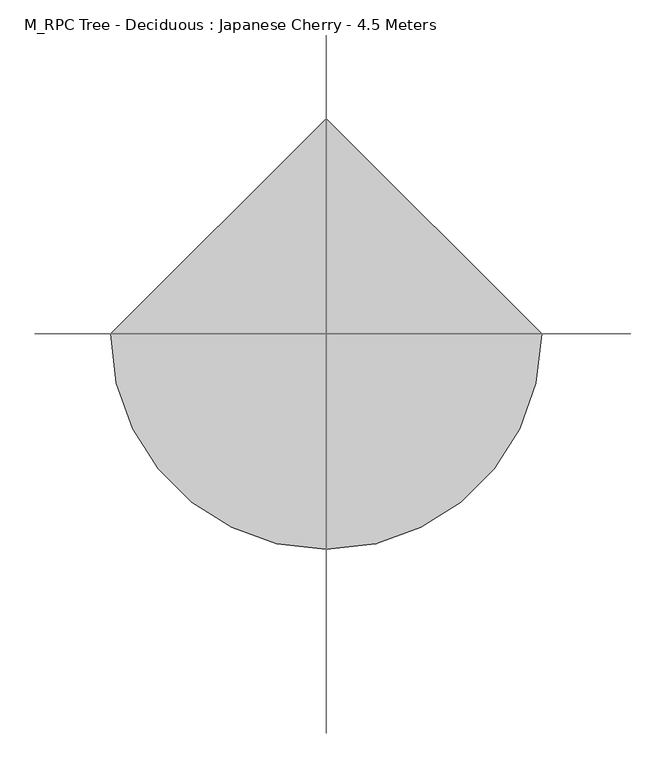
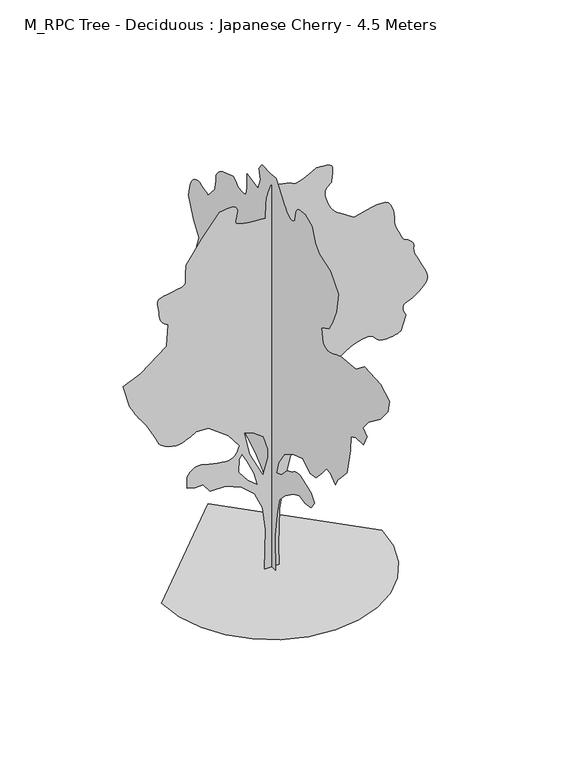
"""IFC4 building model written with IfcOpenShell, lengths in millimetres: geographic element geometry, M_RPC Tree - Deciduous : Japanese Cherry - 4.5 Meters."""

from ifc_helpers import new_model, si_unit, origin, place, context, project, spatial, triangles, source, transform, mapped, element, save


def m_rpc_tree_deciduous_japanese_cherry_4_5_meters_cd2ce576(model_context):
    return source(origin(), model_context, "Body", "Tessellation", [
        triangles([(-0.0027587, 74.5725603, 0.00586), (-0.0027587, -72.0943095, 0.00586), (-0.0027587, -58.7610481, 393.3378007), (-0.0027587, -98.7608322, 653.338028), (-0.0027587, -145.4276149, 853.3381748), (-0.0027587, -252.0952047, 966.670792), (-0.0027587, -412.0928332, 1080.00588), (-0.0027587, -518.7604139, 1126.6709095), (-0.0027587, -625.428031, 1106.6708948), (-0.0027587, -738.7605755, 1126.6709095), (-0.0027587, -798.7606195, 1213.3384392), (-0.0027587, -738.7605755, 1293.3384979), (-0.0027587, -525.4279212, 1366.6710857), (-0.0027587, -506.885412, 1365.1761189), (-0.0027587, -488.5178922, 1363.2711479), (-0.0027587, -470.5003873, 1360.5486397), (-0.0027587, -453.0078504, 1356.6035316), (-0.0027587, -436.2153434, 1351.0261105), (-0.0027587, -420.2953485, 1343.4060814), (-0.0027587, -405.4278331, 1333.3385273), (-0.0027587, -390.5578105, 1322.4935497), (-0.0027587, -374.6402864, 1312.6960373), (-0.0027587, -357.8477795, 1303.7760876), (-0.0027587, -340.3552789, 1295.553479), (-0.0027587, -322.337774, 1287.8585999), (-0.0027587, -303.970236, 1280.5110832), (-0.0027587, -285.4277268, 1273.3385559), (-0.0027587, -185.427399, 1166.6709389), (-0.0027587, -85.4275708, 1126.6709095), (-0.0027587, -125.4276002, 1266.671085), (-0.0027587, -238.7606988, 1433.3386734), (-0.0027587, -398.7603258, 1533.3386742), (-0.0027587, -585.4279653, 1593.3387909), (-0.0027587, -718.7605608, 1506.6712612), (-0.0027587, -825.4281778, 1520.0062031), (-0.0027587, -938.7607224, 1640.0038204), (-0.0027587, -1025.4283247, 1746.6714375), (-0.0027587, -1105.4259127, 1740.0038212), (-0.0027587, -1192.0934423, 1660.0063786), (-0.0027587, -1245.4260155, 1753.3389084), (-0.0027587, -1305.4259869, 1820.0040253), (-0.0027587, -1412.0936039, 1933.3391132), (-0.0027587, -1478.7587208, 2233.3392609), (-0.0027587, -1485.4261917, 2393.3393784), (-0.0027587, -1578.7611923, 2433.336937), (-0.0027587, -1725.426368, 2446.6718788), (-0.0027587, -1785.4264847, 2573.3269386), (-0.0027587, -1712.0938969, 2633.3270554), (-0.0027587, -1812.0938976, 2753.3272888), (-0.0027587, -2038.759132, 2926.6774635), (-0.0027587, -2185.4267784, 3100.0023491), (-0.0027587, -2212.0917206, 3240.0025246), (-0.0027587, -2045.4266029, 3333.3276421), (-0.0027587, -1738.758839, 3346.6776993), (-0.0027587, -1585.4263378, 3226.6774658), (-0.0027587, -1292.0935158, 3193.3274666), (-0.0027587, -1252.2485641, 3177.7025482), (-0.0027587, -1213.3384392, 3162.6025978), (-0.0027587, -1176.2909185, 3148.5525833), (-0.0027587, -1142.0459158, 3136.0774727), (-0.0027587, -1111.5309179, 3125.7025246), (-0.0027587, -1085.6808969, 3117.9524162), (-0.0027587, -1065.4258833, 3113.3274078), (-0.0027587, -1047.2933418, 3113.0774231), (-0.0027587, -1028.108321, 3117.0274727), (-0.0027587, -1009.2758223, 3123.652359), (-0.0027587, -992.1908186, 3131.4524643), (-0.0027587, -978.255768, 3138.9025909), (-0.0027587, -968.8682596, 3144.4775414), (-0.0027587, -965.4257372, 3146.6774071), (-0.0027587, -932.0932514, 3306.6775246), (-0.0027587, -1072.0933542, 3380.0027), (-0.0027587, -1138.7609419, 3486.6778748), (-0.0027587, -1212.093457, 3660.003051), (-0.0027587, -1252.0934864, 3880.0029945), (-0.0027587, -1098.7609125, 4053.3281708), (-0.0027587, -898.760693, 4126.6783447), (-0.0027587, -818.7606342, 4200.0032295), (-0.0027587, -758.7605902, 4360.003347), (-0.0027587, -618.7604874, 4413.3285805), (-0.0027587, -595.9604619, 4413.2285866), (-0.0027587, -573.5129585, 4412.5536278), (-0.0027587, -551.7629416, 4410.70345), (-0.0027587, -531.0629333, 4407.1286682), (-0.0027587, -511.7629123, 4401.17845), (-0.0027587, -494.2128934, 4392.3534073), (-0.0027587, -478.7603846, 4380.0035797), (-0.0027587, -466.2228868, 4364.55336), (-0.0027587, -456.8353784, 4347.0035591), (-0.0027587, -450.0728551, 4327.7035744), (-0.0027587, -445.4078419, 4307.0033844), (-0.0027587, -442.3178415, 4285.2535492), (-0.0027587, -440.2753427, 4262.803466), (-0.0027587, -438.7603552, 4240.0034042), (-0.0027587, -427.2553525, 4227.3033073), (-0.0027587, -415.2803204, 4215.6034401), (-0.0027587, -402.3753304, 4205.9034508), (-0.0027587, -388.070317, 4199.1532814), (-0.0027587, -371.9003011, 4196.3784508), (-0.0027587, -353.3952896, 4198.553318), (-0.0027587, -332.0927745, 4206.6784035), (-0.0027587, -310.9852329, 4218.4782646), (-0.0027587, -293.0277353, 4231.0033722), (-0.0027587, -277.6927156, 4244.1034447), (-0.0027587, -264.4552061, 4257.6784882), (-0.0027587, -252.7927094, 4271.5785118), (-0.0027587, -242.1814384, 4285.7285202), (-0.0027587, -232.0939364, 4300.003521), (-0.0027587, -138.7608616, 4426.6786377), (-0.0027587, -78.7608175, 4500.0035225), (-0.0027587, 21.2393172, 4493.3286392), (-0.0027587, 181.2391372, 4500.0035225), (-0.0027587, 241.2389451, 4420.0034637), (-0.0027587, 214.5724224, 4306.6784042), (-0.0027587, 261.2402133, 4180.0032875), (-0.0027587, 467.9053785, 4220.0034622), (-0.0027587, 467.9053785, 4073.3284035), (-0.0027587, 469.4403866, 4050.6283356), (-0.0027587, 471.6178699, 4028.7032204), (-0.0027587, 475.0778695, 4008.4282951), (-0.0027587, 480.4628969, 3990.6282188), (-0.0027587, 488.4103769, 3976.0532364), (-0.0027587, 499.5679081, 3965.5782944), (-0.0027587, 514.5729152, 3960.0030533), (-0.0027587, 531.7154371, 3957.9281799), (-0.0027587, 548.8579227, 3957.2532211), (-0.0027587, 566.0004447, 3957.7281921), (-0.0027587, 583.1429667, 3959.1531052), (-0.0027587, 600.2854886, 3961.2782661), (-0.0027587, 617.4304813, 3963.853109), (-0.0027587, 634.5730396, 3966.6782272), (-0.0027587, 650.2955538, 3982.2281502), (-0.0027587, 666.0780207, 3996.928125), (-0.0027587, 681.9780676, 4009.8782066), (-0.0027587, 698.0505604, 4020.2031578), (-0.0027587, 714.3580679, 4027.0283226), (-0.0027587, 730.9580721, 4029.4781731), (-0.0027587, 747.9055841, 4026.678344), (-0.0027587, 927.9057163, 3966.6782272), (-0.0027587, 953.4457272, 3949.4781143), (-0.0027587, 977.9358021, 3931.9280228), (-0.0027587, 1000.3257872, 3913.6782646), (-0.0027587, 1019.5682899, 3894.3779892), (-0.0027587, 1034.6108311, 3873.6780899), (-0.0027587, 1044.4058001, 3851.2280067), (-0.0027587, 1047.9058044, 3826.6780518), (-0.0027587, 1048.6833733, 3801.5281334), (-0.0027587, 1050.8608566, 3777.4531494), (-0.0027587, 1054.2033125, 3754.253112), (-0.0027587, 1058.4783422, 3731.7530319), (-0.0027587, 1063.4533293, 3709.7529213), (-0.0027587, 1068.895875, 3688.1280785), (-0.0027587, 1074.570892, 3666.6779343), (-0.0027587, 1201.238451, 3526.6777588), (-0.0027587, 1239.7609543, 3543.5528915), (-0.0027587, 1277.9935043, 3558.9278252), (-0.0027587, 1315.641061, 3571.2779434), (-0.0027587, 1352.4135258, 3579.077758), (-0.0027587, 1388.0210907, 3580.8029434), (-0.0027587, 1422.1711864, 3574.9527191), (-0.0027587, 1454.5710983, 3560.0027596), (-0.0027587, 1482.6961258, 3536.9027161), (-0.0027587, 1504.8736965, 3508.1777252), (-0.0027587, 1522.093721, 3474.8027275), (-0.0027587, 1535.3487259, 3437.7026665), (-0.0027587, 1545.6312378, 3397.8027763), (-0.0027587, 1553.9313126, 3356.02771), (-0.0027587, 1561.2387154, 3313.3277), (-0.0027587, 1474.5711857, 3086.677581), (-0.0027587, 1367.9060394, 2940.0022316), (-0.0027587, 1454.5710983, 2700.0020554), (-0.0027587, 1374.5710396, 2573.3269386), (-0.0027587, 1341.9185268, 2561.8270592), (-0.0027587, 1310.4910847, 2549.851918), (-0.0027587, 1281.5110222, 2536.952124), (-0.0027587, 1256.2035553, 2522.6521248), (-0.0027587, 1235.7959347, 2506.4769493), (-0.0027587, 1221.5109055, 2487.9745903), (-0.0027587, 1214.5709948, 2466.6721115), (-0.0027587, 1212.2984591, 2444.0095413), (-0.0027587, 1211.0734612, 2421.694479), (-0.0027587, 1210.7234825, 2399.6744568), (-0.0027587, 1211.0734612, 2377.8868332), (-0.0027587, 1211.9484804, 2356.2718735), (-0.0027587, 1213.1734783, 2334.7768192), (-0.0027587, 1214.5709948, 2313.3368488), (-0.0027587, 1187.9059799, 2206.6717026), (-0.0027587, 1001.2383041, 2226.6717899), (-0.0027587, 985.728277, 2195.3792233), (-0.0027587, 971.4432478, 2164.9017231), (-0.0027587, 959.6057436, 2136.0591522), (-0.0027587, 951.4432331, 2109.6642517), (-0.0027587, 948.1782434, 2086.536739), (-0.0027587, 951.0357725, 2067.4865936), (-0.0027587, 961.2382748, 2053.3392014), (-0.0027587, 977.7782536, 2041.5990749), (-0.0027587, 998.0507807, 2029.6266953), (-0.0027587, 1020.8883402, 2018.0041489), (-0.0027587, 1045.1258142, 2007.3141037), (-0.0027587, 1069.5958323, 1998.1390823), (-0.0027587, 1093.133349, 1991.0640781), (-0.0027587, 1114.5709213, 1986.6716137), (-0.0027587, 1133.9884134, 1982.8416149), (-0.0027587, 1152.3558969, 1977.2640484), (-0.0027587, 1169.8484339, 1970.2290127), (-0.0027587, 1186.6409409, 1962.0266064), (-0.0027587, 1202.9109507, 1952.9491081), (-0.0027587, 1218.828511, 1943.2890873), (-0.0027587, 1234.5710094, 1933.3391132), (-0.0027587, 1387.9061268, 2013.339172), (-0.0027587, 1431.9861397, 2024.5916828), (-0.0027587, 1474.8436981, 2034.7965832), (-0.0027587, 1515.2512608, 2042.9016117), (-0.0027587, 1551.9862278, 2047.8566872), (-0.0027587, 1583.8238194, 2048.6141991), (-0.0027587, 1609.5388195, 2044.1266823), (-0.0027587, 1627.9038322, 2033.339114), (-0.0027587, 1640.0538174, 2017.6916679), (-0.0027587, 1648.351276, 1999.5965515), (-0.0027587, 1653.4438431, 1979.4615887), (-0.0027587, 1655.9713051, 1957.6915512), (-0.0027587, 1656.5738846, 1934.6990593), (-0.0027587, 1655.8938389, 1910.8890301), (-0.0027587, 1654.5713905, 1886.6714676), (-0.0027587, 1631.6563648, 1862.5889259), (-0.0027587, 1608.3912151, 1839.7339256), (-0.0027587, 1584.4262535, 1819.3239796), (-0.0027587, 1559.4112106, 1802.5889545), (-0.0027587, 1532.9962532, 1790.7539211), (-0.0027587, 1504.833728, 1785.038863), (-0.0027587, 1474.5711857, 1786.6714668), (-0.0027587, 1442.5211071, 1793.7065025), (-0.0027587, 1410.0036152, 1802.1439236), (-0.0027587, 1378.1860806, 1810.1114605), (-0.0027587, 1348.2360191, 1815.7489071), (-0.0027587, 1321.3160053, 1817.1864647), (-0.0027587, 1298.5960258, 1812.5614563), (-0.0027587, 1281.2385098, 1800.0039379), (-0.0027587, 1268.1185257, 1783.8339947), (-0.0027587, 1257.0985588, 1769.4114738), (-0.0027587, 1247.8260143, 1756.448893), (-0.0027587, 1239.9560005, 1744.6513573), (-0.0027587, 1233.1334518, 1733.7264427), (-0.0027587, 1227.0110058, 1723.3863762), (-0.0027587, 1221.2385384, 1713.338879), (-0.0027587, 1243.9585178, 1710.3264175), (-0.0027587, 1265.8635761, 1706.3813095), (-0.0027587, 1286.1360306, 1700.5688736), (-0.0027587, 1303.9584892, 1691.9587887), (-0.0027587, 1318.5160309, 1679.6163734), (-0.0027587, 1328.993589, 1662.608836), (-0.0027587, 1334.5710102, 1640.0038204), (-0.0027587, 1336.8460167, 1613.5137222), (-0.0027587, 1338.0710873, 1585.6212387), (-0.0027587, 1338.4210659, 1556.56371), (-0.0027587, 1338.0710873, 1526.5736801), (-0.0027587, 1337.1961407, 1495.8836929), (-0.0027587, 1335.9710701, 1464.7286179), (-0.0027587, 1334.5710102, 1433.3386734), (-0.0027587, 1300.3260075, 1407.8185741), (-0.0027587, 1266.3110779, 1383.4636654), (-0.0027587, 1232.7634163, 1361.4436432), (-0.0027587, 1199.91593, 1342.9210819), (-0.0027587, 1168.0034157, 1329.0634975), (-0.0027587, 1137.2534031, 1321.0360806), (-0.0027587, 1107.9059212, 1320.0060562), (-0.0027587, 1078.5558958, 1323.638538), (-0.0027587, 1047.808354, 1328.6735504), (-0.0027587, 1015.8932962, 1334.873608), (-0.0027587, 983.0458099, 1342.0060215), (-0.0027587, 949.4982937, 1349.8410084), (-0.0027587, 915.4857622, 1358.1386124), (-0.0027587, 881.238216, 1366.6710857), (-0.0027587, 681.2380692, 1320.0060562), (-0.0027587, 447.9053638, 1200.0059681), (-0.0027587, 314.5727683, 1126.6709095), (-0.0027587, 161.2391225, 1000.0058212), (-0.0027587, 67.9058024, 806.6731453), (-0.0027587, 41.2392842, 533.3379398), (-0.0027587, 67.9058024, 260.0052052), (78.9470616, 0.0002511, 0.0), (-81.0528106, 0.0002511, 0.0), (-67.7195538, 0.0002197, 453.3328669), (-101.05258, 0.0001988, 713.3330578), (-187.7193921, 0.0001884, 899.9981901), (-327.7202579, 0.0001884, 1026.6658218), (-501.0528829, 0.0001779, 1099.9984097), (-667.7180368, 0.0001779, 1099.9984097), (-747.7205664, 0.0001779, 1199.9984831), (-834.3856979, 0.0001779, 1199.9984831), (-921.0532276, 0.0001779, 1219.9984978), (-921.0532276, 0.0001674, 1346.6660568), (-903.7932346, 0.0001674, 1369.3085701), (-885.8332117, 0.0001674, 1390.6686035), (-866.4756723, 0.000157, 1409.4636772), (-845.0181885, 0.000157, 1424.411166), (-820.7606575, 0.000157, 1434.2261192), (-793.0056656, 0.000157, 1437.6286732), (-761.0531101, 0.000157, 1433.3335865), (-723.1130568, 0.000157, 1423.7311203), (-679.5755253, 0.000157, 1412.8461742), (-633.0054754, 0.0001674, 1401.8461189), (-585.970483, 0.0001674, 1391.8936741), (-541.032928, 0.0001674, 1384.1585358), (-500.7603862, 0.0001674, 1379.803569), (-467.71789, 0.0001674, 1379.9986153), (-441.4803563, 0.0001674, 1385.9661289), (-419.4403499, 0.0001674, 1397.5311207), (-400.8978044, 0.000157, 1413.7610893), (-385.1527988, 0.000157, 1433.7212082), (-371.5102813, 0.000157, 1456.4811562), (-359.2652802, 0.000157, 1481.1062519), (-347.7202726, 0.000157, 1506.6661743), (-467.71789, 0.0001465, 1666.6662918), (-687.7180515, 0.000136, 1826.6664093), (-821.0531542, 0.000136, 1833.3314095), (-842.5681927, 0.000136, 1820.5039948), (-864.6081991, 0.000136, 1807.851424), (-887.7006849, 0.000136, 1795.5489773), (-912.3632057, 0.000136, 1783.7688824), (-939.1282871, 0.000136, 1772.6913609), (-968.5158102, 0.000136, 1762.4864605), (-1001.0532864, 0.0001465, 1753.3313507), (-1038.4858126, 0.0001465, 1750.1639568), (-1080.1183731, 0.0001465, 1756.5589153), (-1122.8008696, 0.000136, 1770.6488983), (-1163.385965, 0.000136, 1790.5713741), (-1198.7209448, 0.000136, 1814.4590149), (-1225.6584721, 0.000136, 1840.4465275), (-1241.0509918, 0.000136, 1866.6664387), (-1254.4834568, 0.000136, 1899.3564491), (-1275.8434902, 0.0001256, 1942.8940533), (-1302.4510231, 0.0001256, 1992.6141289), (-1331.6261318, 0.0001256, 2043.8466122), (-1360.6836605, 0.0001256, 2091.9316132), (-1386.9410694, 0.0001151, 2132.204155), (-1407.7185802, 0.0001151, 2159.9992607), (-1425.2510857, 0.0001151, 2182.1367176), (-1443.4812229, 0.0001151, 2208.1242302), (-1462.2962082, 0.0001151, 2237.3167797), (-1481.576136, 0.0001151, 2269.0742889), (-1501.2061878, 0.0001046, 2302.7592968), (-1521.0712543, 0.0001046, 2337.7243137), (-1541.0512848, 0.0001046, 2373.3318787), (-1614.3863434, 9.42e-05, 2626.6771706), (-1421.0511967, 8.37e-05, 2706.6772293), (-1141.0533892, 7.32e-05, 2926.6774635), (-1127.7183746, 5.23e-05, 3166.6526413), (-1147.5834412, 5.23e-05, 3181.0776329), (-1166.6308977, 5.23e-05, 3196.1775833), (-1184.0459684, 5.23e-05, 3212.6774483), (-1199.0109707, 5.23e-05, 3231.2774757), (-1210.7109833, 5.23e-05, 3252.677623), (-1218.3309397, 5.23e-05, 3277.5775566), (-1221.0535206, 5.23e-05, 3306.6525261), (-1223.4635479, 4.19e-05, 3339.402562), (-1228.9034775, 4.19e-05, 3373.552803), (-1234.6960018, 4.19e-05, 3407.2527809), (-1238.155965, 4.19e-05, 3438.6026115), (-1236.6009727, 4.19e-05, 3465.7526985), (-1227.3484852, 4.19e-05, 3486.8278656), (-1207.7184334, 4.19e-05, 3500.0029335), (-1173.335939, 4.19e-05, 3508.2777191), (-1126.1258846, 3.14e-05, 3516.4528015), (-1072.8508661, 3.14e-05, 3525.1778503), (-1020.2758049, 3.14e-05, 3535.2278183), (-975.1632969, 3.14e-05, 3547.2279579), (-944.2782635, 3.14e-05, 3561.9279327), (-934.3857714, 3.14e-05, 3580.0029922), (-936.4657316, 3.14e-05, 3601.7528275), (-937.1457773, 3.14e-05, 3626.6527611), (-936.6582344, 3.14e-05, 3654.1778252), (-935.2407337, 3.14e-05, 3683.7780533), (-933.1232758, 2.09e-05, 3714.9778931), (-930.5382591, 2.09e-05, 3747.2279594), (-927.7182278, 2.09e-05, 3780.0029938), (-761.0531101, 1.05e-05, 4020.00317), (-567.7204705, -1.05e-05, 4260.0033463), (-526.5729095, -1.05e-05, 4266.8535095), (-487.1179049, -1.05e-05, 4272.0284843), (-451.042854, -1.05e-05, 4273.8283745), (-420.0428204, -1.05e-05, 4270.5282852), (-395.80531, -1.05e-05, 4260.4783173), (-380.0228067, -1.05e-05, 4241.9782837), (-374.3852875, 0.0, 4213.3282883), (-377.165314, 0.0, 4181.0532234), (-383.5603088, 0.0, 4152.6032158), (-390.6552973, 0.0, 4127.8032761), (-395.5328339, 0.0, 4106.3534225), (-395.2803057, 0.0, 4088.0533768), (-386.9803036, 0.0, 4072.6781525), (-367.7202873, 0.0, 4060.0033447), (-338.5077536, 0.0, 4049.7280998), (-302.995241, 0.0, 4041.5783066), (-262.2377179, 1.05e-05, 4035.1531174), (-217.282177, 1.05e-05, 4030.1531319), (-169.1771373, 1.05e-05, 4026.1780838), (-118.9730978, 1.05e-05, 4022.9032837), (-67.7195538, 1.05e-05, 4020.00317), (-61.0525507, 0.0, 4200.0032295), (-59.4975493, -1.05e-05, 4225.5284157), (-55.1437952, -1.05e-05, 4250.678334), (-48.4577889, -1.05e-05, 4275.5535599), (-39.9057809, -1.05e-05, 4300.2035088), (-29.954274, -1.05e-05, 4324.6784683), (-19.070066, -1.05e-05, 4349.0284355), (-7.719256, -1.05e-05, 4373.3284058), (37.7812808, -1.05e-05, 4364.7283493), (81.9990646, -1.05e-05, 4356.0285896), (123.6511007, -1.05e-05, 4347.103553), (161.4548797, -1.05e-05, 4337.8035393), (194.127413, -1.05e-05, 4328.053553), (220.3859302, -1.05e-05, 4317.7033127), (238.9474425, -1.05e-05, 4306.6534058), (263.1077047, -1.05e-05, 4303.4283119), (302.4252358, -1.05e-05, 4313.503569), (350.0252918, -1.05e-05, 4332.2035904), (399.0253169, -1.05e-05, 4354.8783691), (442.5428641, -1.05e-05, 4376.8284828), (473.6978665, -2.09e-05, 4393.4286324), (485.6128733, -2.09e-05, 4400.0035217), (495.2154121, -2.09e-05, 4400.2035095), (519.9779268, -2.09e-05, 4399.9285263), (553.8354532, -2.09e-05, 4397.9036499), (590.7254617, -2.09e-05, 4392.8533768), (624.5830244, -1.05e-05, 4383.4783676), (649.3455391, -1.05e-05, 4368.5034096), (658.9480053, -1.05e-05, 4346.6535805), (658.5580582, -1.05e-05, 4321.3283821), (657.4705519, -1.05e-05, 4296.7034317), (655.7980522, -1.05e-05, 4272.6784447), (653.6605373, -1.05e-05, 4249.1034302), (651.1730438, -1.05e-05, 4225.8783943), (648.4505356, 0.0, 4202.8783447), (645.6129908, 0.0, 4180.0032875), (628.6255102, 0.0, 4167.0032089), (612.5730017, 0.0, 4153.2784653), (598.3829885, 0.0, 4138.0032349), (586.992986, 0.0, 4120.4784325), (579.3354592, 0.0, 4099.9282333), (576.3429457, 0.0, 4075.5782661), (578.9479465, 0.0, 4046.6532875), (586.2154535, 1.05e-05, 4014.6032089), (596.2829713, 1.05e-05, 3981.953167), (608.6854846, 1.05e-05, 3949.7530975), (622.9504932, 1.05e-05, 3919.0782257), (638.6155254, 1.05e-05, 3890.9781967), (655.2155296, 1.05e-05, 3866.477948), (672.280549, 2.09e-05, 3846.6529953), (692.3380457, 2.09e-05, 3828.5529373), (717.6455853, 2.09e-05, 3808.6779877), (747.3230616, 2.09e-05, 3787.3531265), (780.5031584, 2.09e-05, 3764.8780449), (816.3031534, 2.09e-05, 3741.5030182), (853.853187, 2.09e-05, 3717.5780251), (892.2807106, 2.09e-05, 3693.3280518), (959.140801, 2.09e-05, 3711.6280975), (1024.3108057, 2.09e-05, 3728.2279564), (1086.098386, 2.09e-05, 3741.4280228), (1142.8159269, 2.09e-05, 3749.5781067), (1192.7659304, 2.09e-05, 3750.9530228), (1234.2634701, 2.09e-05, 3743.8778732), (1265.613446, 2.09e-05, 3726.6530525), (1288.19855, 2.09e-05, 3698.6530174), (1305.0685959, 3.14e-05, 3662.6028923), (1317.0411209, 3.14e-05, 3621.8777618), (1324.9335171, 3.14e-05, 3579.8779999), (1329.5585255, 3.14e-05, 3539.9778191), (1331.7360088, 4.19e-05, 3505.5528854), (1332.2810337, 4.19e-05, 3480.0027008), (1337.451067, 4.19e-05, 3452.7526199), (1350.7835381, 4.19e-05, 3414.6526199), (1369.01353, 4.19e-05, 3371.2026558), (1388.8785965, 5.23e-05, 3327.8526855), (1407.1110592, 5.23e-05, 3290.1026642), (1420.4436756, 5.23e-05, 3263.4275482), (1425.6137089, 5.23e-05, 3253.3275833), (1432.59119, 5.23e-05, 3250.552462), (1450.4136486, 5.23e-05, 3242.5276611), (1474.4187241, 5.23e-05, 3229.7275703), (1499.938678, 5.23e-05, 3212.6024529), (1522.3086788, 5.23e-05, 3191.6275703), (1536.8662205, 5.23e-05, 3167.2776031), (1538.9461807, 6.28e-05, 3140.0025238), (1536.3412525, 6.28e-05, 3112.1024826), (1539.3362732, 6.28e-05, 3085.0273911), (1546.9938, 6.28e-05, 3057.9525902), (1558.3838024, 6.28e-05, 3030.0775475), (1572.5713085, 6.28e-05, 3000.5523148), (1588.6262878, 7.32e-05, 2968.5772316), (1605.6137684, 7.32e-05, 2933.3273483), (1625.0112762, 7.32e-05, 2895.102356), (1646.5088013, 7.32e-05, 2855.2271736), (1666.4888317, 7.32e-05, 2814.5523308), (1681.3363266, 8.37e-05, 2773.8771973), (1687.4413319, 8.37e-05, 2734.0023056), (1681.1813942, 8.37e-05, 2695.7770226), (1658.9462688, 8.37e-05, 2660.0021713), (1628.9963528, 9.42e-05, 2628.8270393), (1601.3762363, 9.42e-05, 2603.2521469), (1575.1563251, 9.42e-05, 2582.3269707), (1549.4036819, 9.42e-05, 2565.1521469), (1523.1837708, 9.42e-05, 2550.7771523), (1495.5661251, 9.42e-05, 2538.2520447), (1465.6137383, 9.42e-05, 2526.6768791), (1440.211219, 9.42e-05, 2513.3021141), (1425.6512066, 9.42e-05, 2496.4220398), (1420.1311947, 9.42e-05, 2476.6369102), (1421.8435902, 0.0001046, 2454.5170395), (1428.976149, 0.0001046, 2430.6494556), (1439.7236034, 0.0001046, 2405.616972), (1452.2811218, 0.0001046, 2379.9993496), (1398.9461506, 0.0001151, 2213.3317612), (1380.1910454, 0.0001151, 2204.8392563), (1360.3261242, 0.0001151, 2196.811694), (1338.2460766, 0.0001151, 2189.7167782), (1312.8435574, 0.0001151, 2184.021777), (1283.0084599, 0.0001151, 2180.194249), (1247.6334389, 0.0001151, 2178.6968113), (1205.6134747, 0.0001151, 2179.9992027), (1167.8684675, 0.0001151, 2188.6467854), (1142.0184465, 0.0001151, 2205.9268353), (1121.9983749, 0.0001151, 2227.4043034), (1101.7459047, 0.0001151, 2248.6467567), (1075.1958538, 0.0001151, 2265.2268494), (1036.2833307, 0.0001151, 2272.7093868), (978.9457695, 0.0001151, 2266.6642616), (912.6507608, 0.0001151, 2247.8318356), (851.8331795, 0.0001151, 2221.3017689), (797.8981722, 0.0001151, 2189.1717533), (752.2405666, 0.0001151, 2153.5467476), (716.2655823, 0.0001151, 2116.5192112), (691.365576, 0.0001256, 2080.1941029), (678.94802, 0.0001256, 2046.6666435), (678.6755075, 0.0001256, 2016.7915775), (688.1980368, 0.0001256, 1989.7166313), (705.8855473, 0.0001256, 1964.9741009), (730.1031097, 0.0001256, 1942.0990437), (759.2181204, 0.000136, 1920.6215755), (791.6006641, 0.000136, 1900.0764633), (825.6131956, 0.000136, 1879.9990551), (845.4582052, 0.000136, 1867.0540604), (864.3707136, 0.000136, 1853.5839523), (881.4156761, 0.000136, 1839.0665245), (895.6632076, 0.000136, 1822.9739021), (906.1781908, 0.000136, 1804.7814079), (912.0281971, 0.000136, 1783.9639286), (912.2807253, 0.000136, 1759.998967), (909.6182425, 0.0001465, 1730.7863605), (907.3057383, 0.0001465, 1695.2763187), (905.28326, 0.0001465, 1654.5187775), (903.4957237, 0.0001465, 1609.5613472), (901.880706, 0.000157, 1561.4562893), (900.3857391, 0.000157, 1511.253685), (898.9457108, 0.000157, 1459.998674), (864.6231691, 0.000157, 1434.5760979), (830.0656855, 0.000157, 1410.9035603), (795.0406431, 0.0001674, 1390.7286289), (759.3156435, 0.0001674, 1375.8010517), (722.6606134, 0.0001674, 1367.8711578), (684.835524, 0.0001674, 1368.686079), (645.6129908, 0.0001674, 1379.9986153), (606.1979911, 0.0001674, 1395.0036587), (567.8304565, 0.0001674, 1406.1611172), (530.3354342, 0.000157, 1414.111068), (493.5429125, 0.000157, 1419.4935883), (457.2753588, 0.000157, 1422.9536968), (421.35782, 0.000157, 1425.1311802), (385.6127998, 0.000157, 1426.6661156), (272.280219, 0.0001674, 1353.3335278), (198.9474132, 0.0001779, 1186.6659393), (125.6138534, 0.0001884, 906.6657337), (85.6140693, 0.0002093, 633.332999), (72.2805581, 0.0002302, 233.3331777), (-94.386072, 8.37e-05, 1079.998395), (-41.0527812, 7.32e-05, 1266.6659981), (-41.0527812, 6.28e-05, 1359.9985279), (-87.7190734, 5.23e-05, 1519.9986454), (-207.7189163, 5.23e-05, 1606.6663204), (-301.052736, 5.23e-05, 1639.9988789), (-241.0526919, 6.28e-05, 1373.3336151), (-154.3856164, 6.28e-05, 993.3332634), (-194.385664, 6.28e-05, 1139.998439), (-267.7202139, 5.23e-05, 1299.9985565), (-321.0527507, 4.19e-05, 1399.9985573), (-354.3852728, 4.19e-05, 1353.3335278), (-361.0527801, 5.23e-05, 1206.665954), (-261.0527066, 6.28e-05, 1079.998395), (-1193.8159389, 0.0, 0.0045206), (-1162.2559467, -273.5427146, 0.0045206), (-1072.3708809, -524.7504189, 0.0045206), (-931.360738, -746.420573, 0.0045206), (-746.420573, -931.360738, 0.0045206), (-524.7504189, -1072.3708809, 0.0045206), (-273.5427146, -1162.2559467, 0.0045206), (5.22e-05, -1193.8159389, 0.0045206), (273.5427146, -1162.2559467, 0.0045206), (524.7504189, -1072.3708809, 0.0045206), (746.420573, -931.360738, 0.0045206), (931.360738, -746.420573, 0.0045206), (1072.3708809, -524.7504189, 0.0045206), (1162.2559467, -273.5427146, 0.0045206), (1193.8159389, 0.0001046, 0.0045206), (-0.0001566, 1193.8159389, 0.0045206)], [[38, 39, 40], [115, 116, 117], [1, 2, 3], [280, 1, 3], [279, 280, 3], [279, 3, 4], [278, 279, 4], [278, 4, 5], [186, 187, 188], [277, 278, 5], [46, 47, 48], [45, 46, 48], [277, 5, 6], [185, 186, 188], [10, 11, 12], [9, 10, 12], [9, 12, 13], [8, 9, 13], [8, 13, 14], [8, 14, 15], [8, 15, 16], [8, 16, 17], [8, 17, 18], [8, 18, 19], [8, 19, 20], [8, 20, 21], [7, 8, 21], [7, 21, 22], [7, 22, 23], [7, 23, 24], [7, 24, 25], [7, 25, 26], [6, 7, 26], [6, 26, 27], [6, 27, 28], [277, 6, 28], [277, 28, 29], [51, 52, 53], [50, 51, 53], [50, 53, 54], [50, 54, 55], [49, 50, 55], [49, 55, 56], [48, 49, 56], [48, 56, 57], [45, 48, 57], [44, 45, 57], [44, 57, 58], [44, 58, 59], [44, 59, 60], [44, 60, 61], [44, 61, 62], [44, 62, 63], [276, 277, 29], [276, 29, 30], [184, 185, 188], [183, 184, 188], [44, 63, 64], [115, 117, 118], [111, 112, 113], [111, 113, 114], [182, 183, 188], [109, 110, 111], [109, 111, 114], [108, 109, 114], [108, 114, 115], [107, 108, 115], [106, 107, 115], [105, 106, 115], [104, 105, 115], [115, 118, 119], [170, 171, 172], [170, 172, 173], [170, 173, 174], [170, 174, 175], [74, 75, 76], [74, 76, 77], [73, 74, 77], [72, 73, 77], [71, 72, 77], [258, 259, 260], [181, 182, 188], [78, 79, 80], [170, 175, 176], [103, 104, 115], [78, 80, 81], [44, 64, 65], [275, 276, 30], [275, 30, 31], [274, 275, 31], [78, 81, 82], [78, 82, 83], [78, 83, 84], [78, 84, 85], [78, 85, 86], [78, 86, 87], [78, 87, 88], [78, 88, 89], [78, 89, 90], [78, 90, 91], [78, 91, 92], [78, 92, 93], [78, 93, 94], [78, 94, 95], [78, 95, 96], [71, 77, 78], [71, 78, 96], [71, 96, 97], [71, 97, 98], [71, 98, 99], [71, 99, 100], [115, 119, 120], [180, 181, 188], [38, 40, 41], [223, 224, 225], [33, 34, 35], [33, 35, 36], [33, 36, 37], [102, 103, 115], [179, 180, 188], [44, 65, 66], [170, 176, 177], [71, 100, 101], [43, 44, 66], [42, 43, 66], [41, 42, 66], [38, 41, 66], [37, 38, 66], [33, 37, 66], [33, 66, 67], [33, 67, 68], [33, 68, 69], [33, 69, 70], [32, 33, 70], [31, 32, 70], [274, 31, 70], [273, 274, 70], [273, 70, 71], [273, 71, 101], [273, 101, 102], [273, 102, 115], [273, 115, 120], [273, 120, 121], [273, 121, 122], [273, 122, 123], [273, 123, 124], [273, 124, 125], [273, 125, 126], [273, 126, 127], [273, 127, 128], [273, 128, 129], [273, 129, 130], [273, 130, 131], [272, 273, 131], [271, 272, 131], [270, 271, 131], [269, 270, 131], [268, 269, 131], [268, 131, 132], [268, 132, 133], [268, 133, 134], [167, 168, 169], [257, 258, 260], [257, 260, 261], [256, 257, 261], [256, 261, 262], [255, 256, 262], [255, 262, 263], [254, 255, 263], [254, 263, 264], [254, 264, 265], [254, 265, 266], [254, 266, 267], [254, 267, 268], [253, 254, 268], [252, 253, 268], [251, 252, 268], [250, 251, 268], [249, 250, 268], [248, 249, 268], [247, 248, 268], [246, 247, 268], [245, 246, 268], [166, 167, 169], [165, 166, 169], [164, 165, 169], [163, 164, 169], [162, 163, 169], [161, 162, 169], [160, 161, 169], [159, 160, 169], [158, 159, 169], [157, 158, 169], [156, 157, 169], [155, 156, 169], [154, 155, 169], [154, 169, 170], [154, 170, 177], [153, 154, 177], [153, 177, 178], [153, 178, 179], [153, 179, 188], [222, 223, 225], [222, 225, 226], [221, 222, 226], [220, 221, 226], [219, 220, 226], [218, 219, 226], [217, 218, 226], [216, 217, 226], [215, 216, 226], [214, 215, 226], [213, 214, 226], [212, 213, 226], [212, 226, 227], [212, 227, 228], [212, 228, 229], [212, 229, 230], [212, 230, 231], [211, 212, 231], [211, 231, 232], [211, 232, 233], [210, 211, 233], [209, 210, 233], [209, 233, 234], [209, 234, 235], [209, 235, 236], [209, 236, 237], [209, 237, 238], [209, 238, 239], [209, 239, 240], [208, 209, 240], [208, 240, 241], [207, 208, 241], [206, 207, 241], [206, 241, 242], [205, 206, 242], [204, 205, 242], [204, 242, 243], [203, 204, 243], [202, 203, 243], [202, 243, 244], [201, 202, 244], [201, 244, 245], [201, 245, 268], [200, 201, 268], [199, 200, 268], [198, 199, 268], [197, 198, 268], [196, 197, 268], [195, 196, 268], [194, 195, 268], [153, 188, 189], [153, 189, 190], [152, 153, 190], [152, 190, 191], [151, 152, 191], [136, 137, 138], [135, 136, 138], [135, 138, 139], [134, 135, 139], [134, 139, 140], [134, 140, 141], [134, 141, 142], [134, 142, 143], [134, 143, 144], [134, 144, 145], [134, 145, 146], [134, 146, 147], [134, 147, 148], [134, 148, 149], [134, 149, 150], [134, 150, 151], [134, 151, 191], [134, 191, 192], [134, 192, 193], [268, 134, 193], [194, 268, 193], [583, 580, 581], [574, 281, 575], [580, 583, 584], [573, 574, 575], [583, 581, 575], [580, 584, 585], [572, 573, 575], [582, 583, 575], [582, 575, 281], [571, 572, 575], [571, 575, 576], [281, 282, 283], [570, 571, 576], [570, 576, 577], [344, 345, 346], [290, 291, 292], [406, 407, 408], [570, 577, 578], [290, 292, 293], [289, 290, 293], [289, 293, 294], [289, 294, 295], [289, 295, 296], [289, 296, 297], [289, 297, 298], [289, 298, 299], [289, 299, 300], [289, 300, 301], [289, 301, 302], [289, 302, 303], [288, 289, 303], [287, 288, 303], [287, 303, 304], [287, 304, 305], [287, 305, 306], [286, 287, 306], [286, 306, 307], [286, 307, 308], [286, 308, 309], [569, 570, 578], [554, 555, 556], [405, 406, 408], [343, 344, 346], [512, 513, 514], [511, 512, 514], [511, 514, 515], [511, 515, 516], [511, 516, 517], [510, 511, 517], [510, 517, 518], [510, 518, 519], [510, 519, 520], [510, 520, 521], [510, 521, 522], [510, 522, 523], [510, 523, 524], [509, 510, 524], [509, 524, 525], [508, 509, 525], [434, 435, 436], [342, 343, 346], [507, 508, 525], [507, 525, 526], [405, 408, 409], [404, 405, 409], [403, 404, 409], [403, 409, 410], [402, 403, 410], [401, 402, 410], [400, 401, 410], [400, 410, 411], [399, 400, 411], [399, 411, 412], [399, 412, 413], [399, 413, 414], [399, 414, 415], [377, 378, 379], [341, 342, 346], [341, 346, 347], [340, 341, 347], [339, 340, 347], [338, 339, 347], [337, 338, 347], [336, 337, 347], [335, 336, 347], [334, 335, 347], [333, 334, 347], [377, 379, 380], [377, 380, 381], [377, 381, 382], [377, 382, 383], [377, 383, 384], [377, 384, 385], [377, 385, 386], [377, 386, 387], [377, 387, 388], [377, 388, 389], [377, 389, 390], [377, 390, 391], [376, 377, 391], [376, 391, 392], [375, 376, 392], [374, 375, 392], [373, 374, 392], [372, 373, 392], [372, 392, 393], [371, 372, 393], [370, 371, 393], [369, 370, 393], [369, 393, 394], [369, 394, 395], [369, 395, 396], [332, 333, 347], [369, 396, 397], [426, 427, 428], [426, 428, 429], [425, 426, 429], [425, 429, 430], [424, 425, 430], [424, 430, 431], [423, 424, 431], [423, 431, 432], [422, 423, 432], [422, 432, 433], [421, 422, 433], [420, 421, 433], [419, 420, 433], [418, 419, 433], [418, 433, 434], [418, 434, 436], [418, 436, 437], [418, 437, 438], [418, 438, 439], [417, 418, 439], [417, 439, 440], [416, 417, 440], [416, 440, 441], [415, 416, 441], [399, 415, 441], [399, 441, 442], [399, 442, 443], [399, 443, 444], [399, 444, 445], [399, 445, 446], [399, 446, 447], [399, 447, 448], [399, 448, 449], [369, 397, 398], [331, 332, 347], [368, 369, 398], [360, 361, 362], [359, 360, 362], [359, 362, 363], [358, 359, 363], [358, 363, 364], [357, 358, 364], [357, 364, 365], [356, 357, 365], [355, 356, 365], [355, 365, 366], [354, 355, 366], [353, 354, 366], [352, 353, 366], [351, 352, 366], [350, 351, 366], [349, 350, 366], [348, 349, 366], [348, 366, 367], [348, 367, 368], [348, 368, 398], [347, 348, 398], [347, 398, 399], [347, 399, 449], [347, 449, 450], [347, 450, 451], [347, 451, 452], [331, 347, 452], [331, 452, 453], [331, 453, 454], [331, 454, 455], [331, 455, 456], [330, 331, 456], [329, 330, 456], [328, 329, 456], [327, 328, 456], [326, 327, 456], [325, 326, 456], [324, 325, 456], [323, 324, 456], [322, 323, 456], [321, 322, 456], [320, 321, 456], [319, 320, 456], [318, 319, 456], [317, 318, 456], [316, 317, 456], [315, 316, 456], [314, 315, 456], [314, 456, 457], [314, 457, 458], [314, 458, 459], [314, 459, 460], [314, 460, 461], [314, 461, 462], [314, 462, 463], [314, 463, 464], [314, 464, 465], [314, 465, 466], [314, 466, 467], [314, 467, 468], [314, 468, 469], [314, 469, 470], [314, 470, 471], [314, 471, 472], [314, 472, 473], [314, 473, 474], [314, 474, 475], [314, 475, 476], [314, 476, 477], [314, 477, 478], [314, 478, 479], [314, 479, 480], [314, 480, 481], [314, 481, 482], [314, 482, 483], [314, 483, 484], [314, 484, 485], [314, 485, 486], [314, 486, 487], [314, 487, 488], [314, 488, 489], [314, 489, 490], [314, 490, 491], [314, 491, 492], [314, 492, 493], [314, 493, 494], [314, 494, 495], [314, 495, 496], [314, 496, 497], [314, 497, 498], [314, 498, 499], [314, 499, 500], [314, 500, 501], [314, 501, 502], [580, 585, 586], [554, 556, 557], [553, 554, 557], [553, 557, 558], [553, 558, 559], [553, 559, 560], [553, 560, 561], [553, 561, 562], [553, 562, 563], [552, 553, 563], [552, 563, 564], [551, 552, 564], [550, 551, 564], [550, 564, 565], [549, 550, 565], [549, 565, 566], [548, 549, 566], [547, 548, 566], [546, 547, 566], [545, 546, 566], [544, 545, 566], [543, 544, 566], [542, 543, 566], [541, 542, 566], [540, 541, 566], [539, 540, 566], [538, 539, 566], [538, 566, 567], [537, 538, 567], [537, 567, 568], [537, 568, 569], [537, 569, 578], [536, 537, 578], [535, 536, 578], [535, 578, 579], [534, 535, 579], [534, 579, 580], [533, 534, 580], [532, 533, 580], [507, 526, 527], [506, 507, 527], [531, 532, 580], [506, 527, 528], [530, 531, 580], [281, 283, 284], [582, 281, 284], [582, 284, 285], [582, 285, 286], [588, 582, 286], [587, 588, 286], [587, 286, 309], [586, 587, 309], [586, 309, 310], [586, 310, 311], [586, 311, 312], [586, 312, 313], [580, 586, 313], [580, 313, 314], [530, 580, 314], [529, 530, 314], [502, 503, 504], [502, 504, 505], [314, 502, 505], [529, 314, 505], [529, 505, 506], [529, 506, 528], [603, 604, 589], [602, 603, 589], [602, 589, 590], [601, 602, 590], [601, 590, 591], [601, 591, 592], [600, 601, 592], [599, 600, 592], [599, 592, 593], [599, 593, 594], [599, 594, 595], [599, 595, 596], [599, 596, 597], [599, 597, 598]], closed=False),
    ])


if __name__ == "__main__":
    model = new_model("IFC4")
    model_context = context("Model", 3, world=origin())
    ifc_project = project(units=[si_unit("LENGTHUNIT", "METRE", prefix="MILLI")], contexts=[model_context])
    site = spatial("IfcSite", under=ifc_project)
    building = spatial("IfcBuilding", under=site)
    placement = place(None, origin())
    m_rpc_tree_deciduous_japanese_cherry_4_5_meters_shape = m_rpc_tree_deciduous_japanese_cherry_4_5_meters_cd2ce576(model_context)
    element("IfcGeographicElement", 1, ObjectType="M_RPC Tree - Deciduous : Japanese Cherry - 4.5 Meters", at=placement, inside=building, context=model_context, shape_type="MappedRepresentation", body=[
        mapped(m_rpc_tree_deciduous_japanese_cherry_4_5_meters_shape, transform((0.0, 0.0, 0.0), x_axis=(1.0, 0.0, 0.0), y_axis=(0.0, 1.0, 0.0), z_axis=(0.0, 0.0, 1.0))),
    ])
    save(model, "model.ifc")

# Revit data of these elements
# Type "M_RPC Tree - Deciduous : Japanese Cherry - 4.5 Meters"
#   built-in parameter 1005198 = "{2, 15},{39, RPC-16-FXGW-2MQ0-PN7K-A000-ST1L-LVER-AU},{1, 0},{1, 0},{2, 13},{1, 8},{5, Color},{1, 0},{1, 0},{3, 0.8},{3, 0.8},{3, 0.8},{1, 8},{7, BBoxMin},{1, 0},{1, 0},{1, 0},{1, 0},{1, 0},{1, 8},{7, BBoxMax},{1, 0},{1, 0},{1, 0},{1, 0},{1, 0},{2, 11},{9, RPCTypeId},{1, 0},{1, 0},{39, RPC-16-FXGW-2MQ0-PN7K-A000-ST1L-LVER-AU},{1, 6},{14, RPCPlantHeight},{1, 0},{1, 0},{7, 14.7638},{2, 11},{7, keyword},{1, 0},{1, 0},{34, :RPCs:Trees [General]:Geometry:RPC},{2, 11},{8, category},{1, 0},{1, 0},{15, Trees [General]},{2, 11},{12, LocalizedUID},{1, 0},{1, 0},{25, Japanese Flowering Cherry},{2, 14},{6, Height},{1, 0},{1, 0},{7, 14.7638},{1, 2},{16, Cast Reflections},{1, 0},{1, 0},{1, 0},{1, 2},{12, Cast Shadows},{1, 0},{1, 0},{1, 1},{1, 2},{9, Lock View},{1, 0},{1, 0},{1, 0},{1, 4},{5, ViewC},{1, 0},{1, 0},{1, 0},{21, assetlibrary_base.fbx},{1, 5},"
#   built-in parameter 1005195 = "RPC-16-FXGW-2MQ0-PN7K-A000-ST1L-LVER-AU"
#   Type Comments = "Japanese Cherry"
#   Height = 4.50 m
#   Default Elevation = 0
